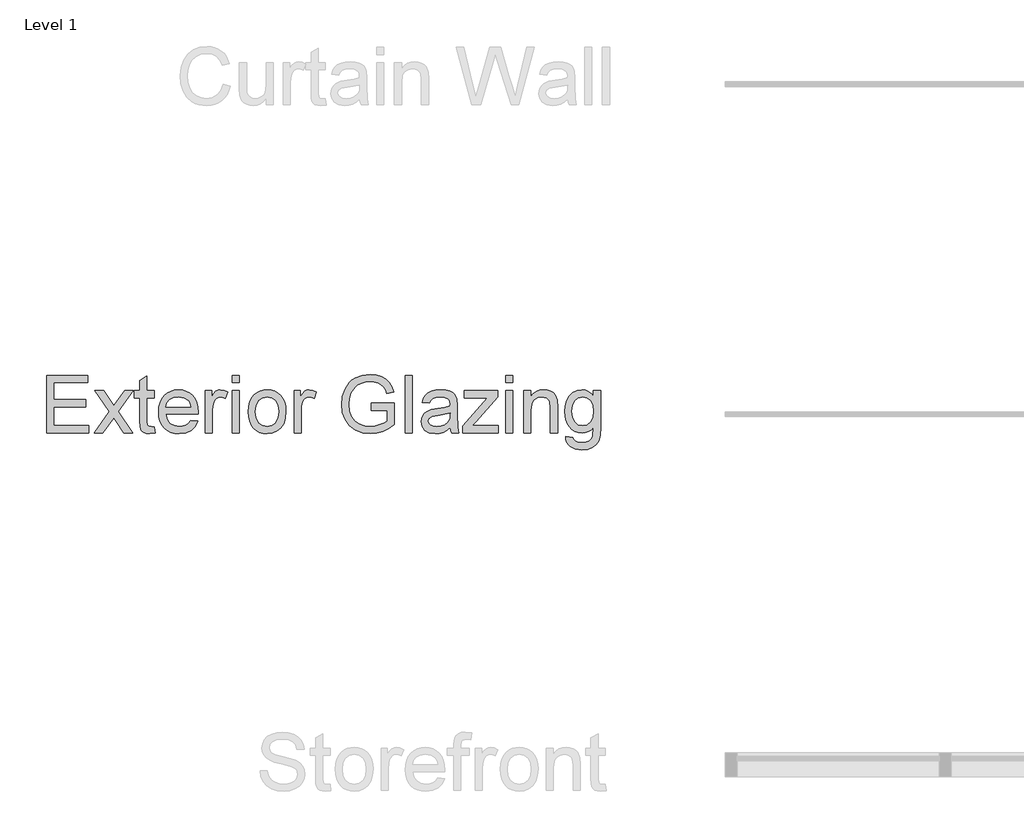
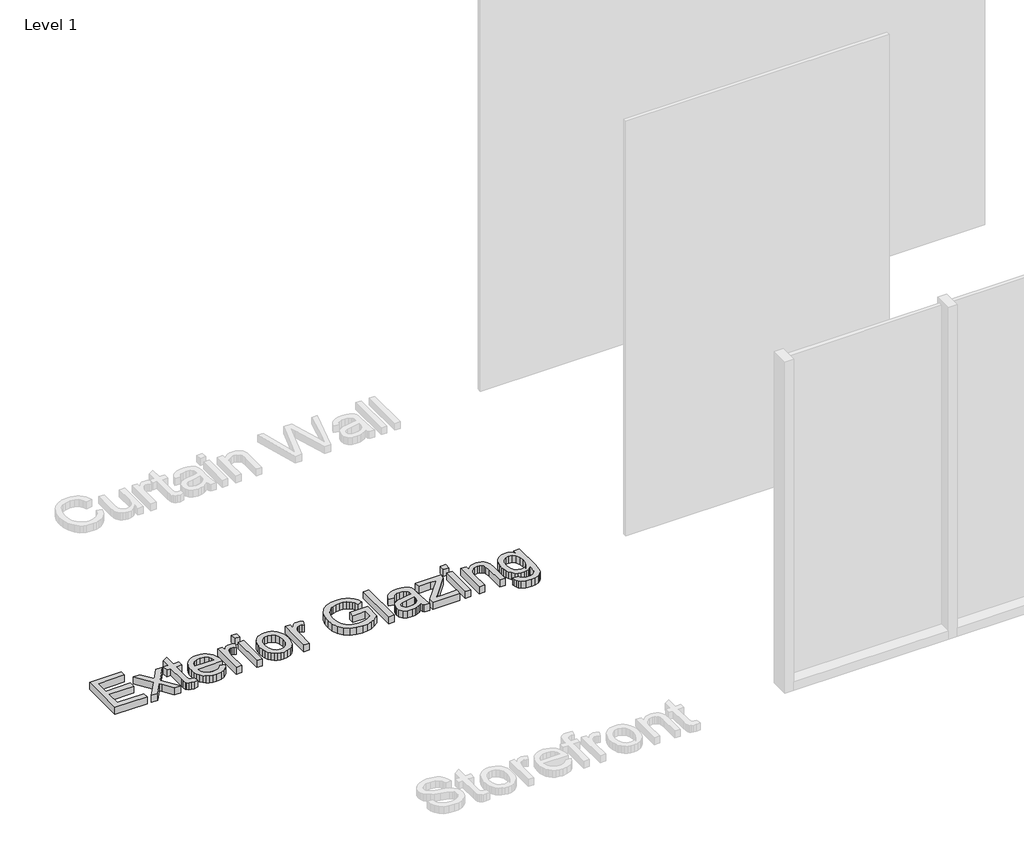
# One storey, part 37 of 42: 1 proxy.
"""IFC4 building model written with IfcOpenShell, lengths in millimetres."""

from ifc_helpers import new_model, si_unit, origin, origin_with_axes, place, context, project, spatial, polyline, outline, extrude, element, save

model = new_model("IFC4")

# Units and contexts
model_context = context("Model", 3, world=origin())
ifc_project = project(units=[si_unit("LENGTHUNIT", "METRE", prefix="MILLI")], contexts=[model_context])

# Site, building, storey
site = spatial("IfcSite", under=ifc_project)
building = spatial("IfcBuilding", under=site)
storey = spatial("IfcBuildingStorey", under=building, Name="Level 1", Elevation=0.0)

# Proxy
placement = place(None, origin())
element("IfcBuildingElementProxy", 1, Name="8\" Arial", ObjectType="8\" Arial", at=placement, inside=storey, context=model_context, shape_type="SweptSolid", body=[
    extrude(outline(polyline([(17706.9887274, 14937.9204205), (17706.9887274, 15242.4875146), (17925.8963263, 15242.4875146), (17925.8963263, 15204.4166278), (17745.0596142, 15204.4166278), (17745.0596142, 15113.9982718), (17916.3786046, 15113.9982718), (17916.3786046, 15075.927385), (17745.0596142, 15075.927385), (17745.0596142, 14975.9913073), (17930.6551871, 14975.9913073), (17930.6551871, 14937.9204205), (17706.9887274, 14937.9204205)])), origin_with_axes(), (0.0, 0.0, 1.0), 50.8),
    extrude(outline(polyline([(17959.2083522, 14937.9204205), (18040.5551298, 15050.348508), (17963.9672131, 15161.5868802), (18009.7712487, 15161.5868802), (18046.7267774, 15108.0496957), (18063.977648, 15082.7682475), (18078.9234453, 15103.4395493), (18121.0096209, 15161.5868802), (18166.8136566, 15161.5868802), (18086.3591654, 15050.348508), (18163.8393685, 14937.9204205), (18118.0353329, 14937.9204205), (18071.4133681, 15005.511116), (18062.86229, 15017.8544113), (18005.0123878, 14937.9204205), (17959.2083522, 14937.9204205)])), origin_with_axes(), (0.0, 0.0, 1.0), 50.8),
    extrude(outline(polyline([(18278.0520288, 14969.6709452), (18282.8108897, 14936.8050625), (18254.3320818, 14933.1615597), (18236.0587997, 14934.7416502), (18222.4328427, 14939.4819217), (18212.8035852, 14946.7875167), (18206.5204017, 14956.0635775), (18203.0627919, 14971.9946077), (18201.9102553, 14999.2651111), (18201.9102553, 15123.5159935), (18173.3570902, 15123.5159935), (18173.3570902, 15161.5868802), (18201.9102553, 15161.5868802), (18201.9102553, 15215.9419939), (18239.981142, 15238.3235114), (18239.981142, 15161.5868802), (18278.0520288, 15161.5868802), (18278.0520288, 15123.5159935), (18239.981142, 15123.5159935), (18239.981142, 15000.3804691), (18241.9887865, 14980.7501681), (18248.4950415, 14973.7977699), (18261.4703731, 14971.2324464), (18278.0520288, 14969.6709452)])), origin_with_axes(), (0.0, 0.0, 1.0), 50.8),
    extrude(outline(polyline([(18472.7191802, 15004.5444724), (18510.046495, 14999.7856115), (18496.5971363, 14971.6600003), (18475.1357893, 14950.6355018), (18446.1457756, 14937.5300452), (18410.1104173, 14933.1615597), (18386.4880641, 14935.04605), (18365.4403289, 14940.6995209), (18346.9672119, 14950.1219724), (18331.0687129, 14963.3134046), (18318.2839217, 14979.9066786), (18309.151928, 14999.534656), (18303.6727318, 15022.1973365), (18301.846333, 15047.8947204), (18303.6913211, 15074.4634776), (18309.2262852, 15097.8813485), (18318.4512254, 15118.1483331), (18331.3661417, 15135.2644312), (18347.2228148, 15148.8625043), (18365.2730252, 15158.5754136), (18385.5167731, 15164.4031592), (18407.9540584, 15166.3457411), (18429.6686847, 15164.4078065), (18449.3059567, 15158.5940029), (18466.8658743, 15148.9043302), (18482.3484377, 15135.3387884), (18494.9868382, 15118.2598689), (18504.0142671, 15098.0300629), (18509.4307244, 15074.6493706), (18511.2362102, 15048.117792), (18511.0131386, 15037.8564983), (18339.9172198, 15037.8564983), (18346.5071267, 15009.3591011), (18361.8154154, 14988.4089598), (18383.9087987, 14975.5265748), (18410.8539893, 14971.2324464), (18431.1163264, 14973.2215016), (18448.181304, 14979.1886669), (18462.0489219, 14989.5057285), (18472.7191802, 15004.5444724)]), holes=[polyline([(18339.9172198, 15075.927385), (18473.1653234, 15075.927385), (18468.0160873, 15096.0410078), (18457.9220973, 15110.4291262), (18435.7264729, 15123.8134223), (18407.805344, 15128.2748543), (18382.1428151, 15124.7150033), (18360.923129, 15114.0354504), (18346.1725193, 15097.3887321), (18339.9172198, 15075.927385)])]), origin_with_axes(), (0.0, 0.0, 1.0), 50.8),
    extrude(outline(polyline([(18549.307097, 14937.9204205), (18549.307097, 15161.5868802), (18582.6191229, 15161.5868802), (18582.6191229, 15128.4979259), (18594.9252396, 15147.6820837), (18606.2647127, 15158.9843782), (18617.6413644, 15164.5054004), (18630.0590169, 15166.3457411), (18649.0201031, 15163.4086317), (18668.2786181, 15154.5973034), (18655.5635368, 15120.4673482), (18642.1792406, 15126.3229778), (18628.7949445, 15128.2748543), (18617.4275875, 15126.397335), (18607.2685349, 15120.7647771), (18599.0613589, 15111.8047344), (18593.5496314, 15099.9447609), (18588.9208956, 15078.6786015), (18587.3779837, 15055.4791548), (18587.3779837, 14937.9204205), (18549.307097, 14937.9204205)])), origin_with_axes(), (0.0, 0.0, 1.0), 50.8),
    extrude(outline(polyline([(18692.0729223, 15204.4166278), (18692.0729223, 15242.4875146), (18730.1438091, 15242.4875146), (18730.1438091, 15204.4166278), (18692.0729223, 15204.4166278)])), origin_with_axes(), (0.0, 0.0, 1.0), 50.8),
    extrude(outline(polyline([(18692.0729223, 14937.9204205), (18692.0729223, 15161.5868802), (18730.1438091, 15161.5868802), (18730.1438091, 14937.9204205), (18692.0729223, 14937.9204205)])), origin_with_axes(), (0.0, 0.0, 1.0), 50.8),
    extrude(outline(polyline([(18777.7324175, 15049.7536504), (18779.7911825, 15078.7204274), (18785.9674775, 15103.6812102), (18796.2613025, 15124.6359988), (18810.6726574, 15141.5847932), (18825.1816062, 15152.4177079), (18841.1962883, 15160.1555041), (18858.7167037, 15164.7981818), (18877.7428525, 15166.3457411), (18898.746438, 15164.4612508), (18917.7377318, 15158.8077799), (18934.7167338, 15149.3853283), (18949.6834441, 15136.1938962), (18961.898938, 15119.6796267), (18970.6242908, 15100.2886629), (18975.8595024, 15078.021005), (18977.604573, 15052.8766528), (18974.5187492, 15014.4153907), (18965.2612777, 14985.137243), (18950.1017034, 14963.2111634), (18929.3095711, 14946.806106), (18904.6136859, 14936.5726963), (18877.7428525, 14933.1615597), (18856.4325435, 14935.039079), (18837.2646513, 14940.671637), (18820.239176, 14950.0592335), (18805.3561176, 14963.2018688), (18793.2707488, 14979.876471), (18784.6383425, 14999.8599687), (18779.4588988, 15023.1523618), (18777.7324175, 15049.7536504)]), holes=[polyline([(18815.8033043, 15049.8280076), (18820.2089684, 15015.3727397), (18833.4259608, 14990.8255688), (18853.316512, 14976.130727), (18877.7428525, 14971.2324464), (18902.0576571, 14976.158611), (18921.9110297, 14990.9371046), (18935.1280221, 15015.8095883), (18939.5336862, 15051.0177228), (18935.1001381, 15084.4691685), (18921.7994939, 15108.6817319), (18901.9182373, 15123.3765737), (18877.7428525, 15128.2748543), (18853.316512, 15123.395163), (18833.4259608, 15108.7560891), (18820.2089684, 15084.2646862), (18815.8033043, 15049.8280076)])]), origin_with_axes(), (0.0, 0.0, 1.0), 50.8),
    extrude(outline(polyline([(19020.4343206, 14937.9204205), (19020.4343206, 15161.5868802), (19053.7463465, 15161.5868802), (19053.7463465, 15128.4979259), (19066.0524632, 15147.6820837), (19077.3919363, 15158.9843782), (19088.768588, 15164.5054004), (19101.1862406, 15166.3457411), (19120.1473267, 15163.4086317), (19139.4058417, 15154.5973034), (19126.6907604, 15120.4673482), (19113.3064643, 15126.3229778), (19099.9221681, 15128.2748543), (19088.5548111, 15126.397335), (19078.3957585, 15120.7647771), (19070.1885825, 15111.8047344), (19064.676855, 15099.9447609), (19060.0481193, 15078.6786015), (19058.5052074, 15055.4791548), (19058.5052074, 14937.9204205), (19020.4343206, 14937.9204205)])), origin_with_axes(), (0.0, 0.0, 1.0), 50.8),
    extrude(outline(polyline([(19429.6963533, 15056.8919416), (19429.6963533, 15094.9628284), (19553.4267352, 15094.9628284), (19553.4267352, 14981.1219541), (19523.3585422, 14960.2089914), (19492.3422948, 14945.2074262), (19460.4523504, 14936.1730263), (19427.763066, 14933.1615597), (19385.0541489, 14937.9483045), (19346.4534671, 14952.3085389), (19314.3869243, 14975.7403517), (19291.2804242, 15007.741832), (19277.3105651, 15046.1287368), (19272.6539454, 15088.7168235), (19277.2919758, 15131.6116337), (19291.2060669, 15171.5135665), (19313.8199506, 15204.9836015), (19328.173214, 15218.0170246), (19344.5573585, 15228.5827181), (19381.996209, 15242.5804611), (19424.7144208, 15247.2463754), (19456.0745702, 15244.5416323), (19484.2745386, 15236.4274027), (19508.0223695, 15223.4892498), (19526.0261068, 15206.3127365), (19539.3453403, 15184.0706388), (19549.0396604, 15155.935733), (19513.9430616, 15146.0462253), (19506.1076716, 15166.1133748), (19496.5806553, 15181.2543598), (19483.9771098, 15192.6681901), (19466.9121322, 15201.5538756), (19446.5661432, 15207.2700854), (19424.1195632, 15209.1754887), (19397.8435874, 15207.121371), (19375.3784181, 15200.959018), (19356.8077073, 15191.4598856), (19342.2151066, 15179.3954298), (19322.6219842, 15150.0615141), (19313.6991202, 15121.3224561), (19310.7248321, 15090.2783248), (19314.3032724, 15053.8711804), (19325.0385933, 15023.9145231), (19342.6054819, 15000.62213), (19366.6786257, 14984.207778), (19394.8507101, 14974.4762793), (19424.7144208, 14971.2324464), (19451.0833431, 14973.6769394), (19476.8016399, 14981.0104183), (19499.1366841, 14991.113703), (19515.3558485, 15001.8676131), (19515.3558485, 15056.8919416), (19429.6963533, 15056.8919416)])), origin_with_axes(), (0.0, 0.0, 1.0), 50.8),
    extrude(outline(polyline([(19610.5330654, 14937.9204205), (19610.5330654, 15242.4875146), (19648.6039521, 15242.4875146), (19648.6039521, 14937.9204205), (19610.5330654, 14937.9204205)])), origin_with_axes(), (0.0, 0.0, 1.0), 50.8),
    extrude(outline(polyline([(19848.4761076, 14966.4735856), (19830.2864774, 14950.8771628), (19811.5577575, 14940.671637), (19791.8623939, 14935.039079), (19770.7728329, 14933.1615597), (19738.9572456, 14937.6787596), (19715.4882541, 14951.2303595), (19701.016484, 14971.8087147), (19696.1925606, 14997.4061811), (19698.014312, 15013.1884969), (19703.4795662, 15027.5208474), (19711.9098139, 15039.7897855), (19722.6265454, 15049.3818644), (19749.2836019, 15061.8738741), (19782.2238418, 15067.5993786), (19821.1498363, 15073.6223118), (19848.253036, 15080.6862459), (19848.4761076, 15089.1629668), (19845.8550163, 15106.1535871), (19837.9917423, 15117.2699886), (19820.4062643, 15125.5236379), (19795.9055667, 15128.2748543), (19773.2266205, 15126.4438083), (19757.3885367, 15120.9506701), (19746.5881533, 15110.7916175), (19739.0223082, 15094.9628284), (19700.9514214, 15099.7216893), (19707.5599176, 15120.5417054), (19717.4215414, 15136.9002896), (19731.456463, 15149.4108886), (19750.5848529, 15158.6869494), (19773.9794871, 15164.4310432), (19800.8131419, 15166.3457411), (19826.550028, 15164.6541148), (19846.951785, 15159.5792358), (19862.3344309, 15151.9483281), (19873.0139838, 15142.5886155), (19880.0965072, 15131.0167761), (19884.6880643, 15116.7494882), (19886.5469944, 15083.4374623), (19886.5469944, 15036.0719255), (19888.4802816, 14969.9311954), (19896.064716, 14937.9204205), (19857.9938293, 14937.9204205), (19851.8965388, 14951.1560023), (19848.4761076, 14966.4735856)]), holes=[polyline([(19848.4761076, 15042.6153591), (19787.0570598, 15030.9412786), (19754.3027129, 15024.7696309), (19739.4684514, 15014.7314089), (19734.2634473, 15000.0830403), (19737.0983156, 14988.7621565), (19745.6029204, 14979.4860957), (19759.5913688, 14973.2958588), (19778.8777677, 14971.2324464), (19799.3259979, 14973.5096357), (19817.3947977, 14980.3412035), (19832.0431662, 14990.4073096), (19842.2301027, 15002.3881135), (19846.7473027, 15014.7314089), (19848.253036, 15031.833565), (19848.4761076, 15042.6153591)])]), origin_with_axes(), (0.0, 0.0, 1.0), 50.8),
    extrude(outline(polyline([(19915.1001594, 14937.9204205), (19915.1001594, 14973.7605913), (20046.4893331, 15123.5159935), (20007.6005171, 15123.5159935), (19924.6178811, 15123.5159935), (19924.6178811, 15161.5868802), (20100.6957324, 15161.5868802), (20100.6957324, 15129.2414979), (19984.1779989, 14996.3651803), (19966.3322707, 14975.9913073), (20010.3517335, 14975.9913073), (20105.4545932, 14975.9913073), (20105.4545932, 14937.9204205), (19915.1001594, 14937.9204205)])), origin_with_axes(), (0.0, 0.0, 1.0), 50.8),
    extrude(outline(polyline([(20143.52548, 15204.4166278), (20143.52548, 15242.4875146), (20181.5963667, 15242.4875146), (20181.5963667, 15204.4166278), (20143.52548, 15204.4166278)])), origin_with_axes(), (0.0, 0.0, 1.0), 50.8),
    extrude(outline(polyline([(20143.52548, 14937.9204205), (20143.52548, 15161.5868802), (20181.5963667, 15161.5868802), (20181.5963667, 14937.9204205), (20143.52548, 14937.9204205)])), origin_with_axes(), (0.0, 0.0, 1.0), 50.8),
    extrude(outline(polyline([(20238.7026969, 14937.9204205), (20238.7026969, 15161.5868802), (20276.7735836, 15161.5868802), (20276.7735836, 15130.3568559), (20289.9998707, 15146.1019932), (20305.8844277, 15157.3485198), (20324.4272546, 15164.0964358), (20345.6283515, 15166.3457411), (20364.39425, 15164.5332843), (20381.580058, 15159.095914), (20395.9124085, 15150.7121396), (20406.1179342, 15140.0604706), (20417.5317646, 15112.0649846), (20419.539409, 15075.2581702), (20419.539409, 14937.9204205), (20381.4685222, 14937.9204205), (20381.4685222, 15070.1275234), (20377.0814474, 15103.8113353), (20371.0120409, 15113.8402627), (20361.577971, 15121.6198849), (20349.4856313, 15126.611112), (20335.441415, 15128.2748543), (20313.1435494, 15124.538405), (20294.13599, 15113.329057), (20286.5399372, 15104.178474), (20281.1141852, 15091.6725223), (20276.7735836, 15056.5945128), (20276.7735836, 14937.9204205), (20238.7026969, 14937.9204205)])), origin_with_axes(), (0.0, 0.0, 1.0), 50.8),
    extrude(outline(polyline([(20462.3691566, 14918.8849771), (20500.4400433, 14914.1261163), (20504.6412252, 14902.2289642), (20512.7833387, 14894.0496721), (20528.7887261, 14887.6921315), (20549.7388674, 14885.5729512), (20572.0832062, 14887.970971), (20588.7020406, 14895.1650301), (20600.2274067, 14906.6903962), (20607.2913407, 14922.0823368), (20609.8938428, 14966.4735856), (20597.2252347, 14953.9815759), (20583.0880719, 14945.0587118), (20567.4823544, 14939.7049933), (20550.4080822, 14937.9204205), (20529.5346218, 14939.9977748), (20511.1567749, 14946.2298377), (20495.2745416, 14956.6166092), (20481.8879218, 14971.1580892), (20471.2664604, 14988.6041475), (20463.6797022, 15007.7046534), (20459.1276474, 15028.459607), (20457.6102957, 15050.8690084), (20460.3336282, 15081.6064162), (20468.5036256, 15109.8714471), (20481.8321539, 15133.8237604), (20500.0310787, 15151.6230153), (20522.4776587, 15162.6650596), (20548.5491522, 15166.3457411), (20566.3530544, 15164.2637395), (20582.5118036, 15158.0177346), (20597.0253997, 15147.6077265), (20609.8938428, 15133.0337152), (20609.8938428, 15161.5868802), (20647.9647295, 15161.5868802), (20647.9647295, 14968.48123), (20645.3622275, 14923.8947935), (20637.5547214, 14894.5329939), (20624.1053628, 14875.060702), (20604.5773029, 14860.1427886), (20579.3980958, 14850.6622455), (20548.9952954, 14847.5020645), (20513.5733839, 14851.9542019), (20485.680139, 14865.310614), (20475.1748607, 14875.3372178), (20467.7879376, 14887.6084796), (20463.5193695, 14902.1243994), (20462.3691566, 14918.8849771)]), holes=[polyline([(20495.6811825, 15053.4715104), (20499.7429446, 15018.55151), (20511.9282308, 14994.5434289), (20530.2479862, 14980.6293377), (20552.7131554, 14975.9913073), (20575.011021, 14980.6014537), (20593.4237228, 14994.4318931), (20605.7763128, 15018.1332508), (20609.8938428, 15052.3561524), (20605.6554823, 15085.3614549), (20592.940401, 15109.1278751), (20574.2581543, 15123.4881095), (20552.1182978, 15128.2748543), (20530.3781113, 15123.5624667), (20512.1513024, 15109.4253039), (20499.7987125, 15086.0120804), (20495.6811825, 15053.4715104)])]), origin_with_axes(), (0.0, 0.0, 1.0), 50.8),
])

save(model, "model.ifc")

# Revit data of these elements
# Element 1 (IfcBuildingElementProxy, "8\" Arial")
#   Phase Created = New Construction
